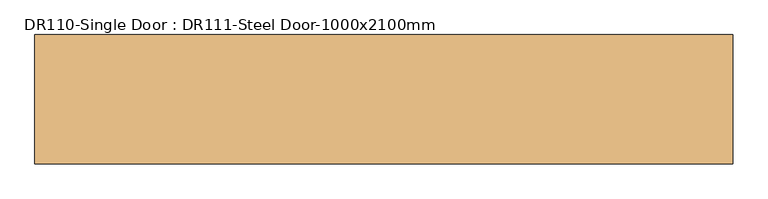
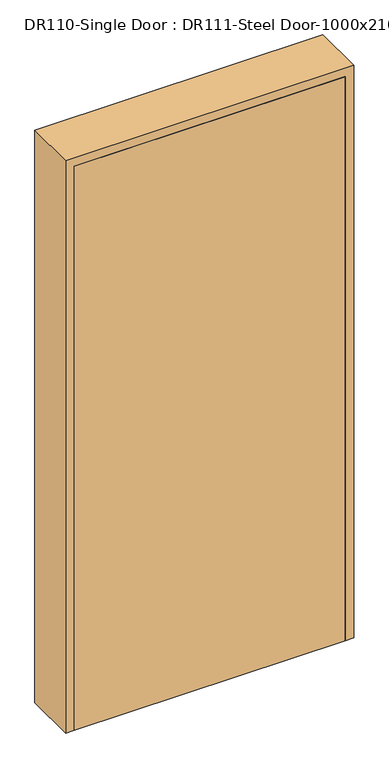
"""IFC4 building model written with IfcOpenShell, lengths in millimetres: door geometry, DR110-Single Door : DR111-Steel Door-1000x2100mm."""

from ifc_helpers import new_model, si_unit, origin, origin_with_axes, place, context, project, spatial, polyline, outline, extrude, faceted_brep, source, transform, mapped, element, save


def dr110_single_door_dr111_steel_door_1000x2100mm_67953bf6(model_context):
    return source(origin(), model_context, "Body", "SolidModel", [
        extrude(outline(polyline([(470.0, -92.5), (-470.0, -92.5), (-470.0, -57.5), (470.0, -57.5), (470.0, -92.5)])), origin_with_axes(), (0.0, 0.0, 1.0), 2070.0),
        faceted_brep([(470.0, -92.5, 0.0), (470.0, -57.5, 0.0), (450.0, -57.5, 0.0), (450.0, 57.5, 0.0), (470.0, 57.5, 0.0), (470.0, 92.5, 0.0), (500.0, 92.5, 0.0), (500.0, -92.5, 0.0), (500.0, -92.5, 2100.0), (-500.0, -92.5, 2100.0), (-500.0, -92.5, 0.0), (-470.0, -92.5, 0.0), (-470.0, -92.5, 2070.0), (470.0, -92.5, 2070.0), (500.0, 92.5, 2100.0), (470.0, 92.5, 2070.0), (-470.0, 92.5, 2070.0), (-470.0, 92.5, 0.0), (-500.0, 92.5, 0.0), (-500.0, 92.5, 2100.0), (470.0, 57.5, 2070.0), (450.0, 57.5, 2050.0), (-450.0, 57.5, 2050.0), (-450.0, 57.5, 0.0), (-470.0, 57.5, 0.0), (-470.0, 57.5, 2070.0), (450.0, -57.5, 2050.0), (470.0, -57.5, 2070.0), (-470.0, -57.5, 2070.0), (-470.0, -57.5, 0.0), (-450.0, -57.5, 0.0), (-450.0, -57.5, 2050.0)], [[[0, 1, 2, 3, 4, 5, 6, 7]], [[7, 8, 9, 10, 11, 12, 13, 0]], [[6, 14, 8, 7]], [[5, 15, 16, 17, 18, 19, 14, 6]], [[4, 20, 15, 5]], [[3, 21, 22, 23, 24, 25, 20, 4]], [[2, 26, 21, 3]], [[1, 27, 28, 29, 30, 31, 26, 2]], [[0, 13, 27, 1]], [[12, 11, 29, 28]], [[11, 10, 18, 17, 24, 23, 30, 29]], [[19, 18, 10, 9]], [[25, 24, 17, 16]], [[31, 30, 23, 22]], [[14, 19, 9, 8]], [[20, 25, 16, 15]], [[26, 31, 22, 21]], [[13, 12, 28, 27]]]),
    ])


if __name__ == "__main__":
    model = new_model("IFC4")
    model_context = context("Model", 3, world=origin())
    ifc_project = project(units=[si_unit("LENGTHUNIT", "METRE", prefix="MILLI")], contexts=[model_context])
    site = spatial("IfcSite", under=ifc_project)
    building = spatial("IfcBuilding", under=site)
    placement = place(None, origin())
    dr110_single_door_dr111_steel_door_1000x2100mm_shape = dr110_single_door_dr111_steel_door_1000x2100mm_67953bf6(model_context)
    element("IfcDoor", 1, ObjectType="DR110-Single Door : DR111-Steel Door-1000x2100mm", at=placement, inside=building, context=model_context, shape_type="MappedRepresentation", body=[
        mapped(dr110_single_door_dr111_steel_door_1000x2100mm_shape, transform((0.0, 0.0, 0.0), x_axis=(1.0, 0.0, 0.0), y_axis=(0.0, 1.0, 0.0), z_axis=(0.0, 0.0, 1.0))),
    ])
    save(model, "model.ifc")

# Revit data of these elements
# Type "DR110-Single Door : DR111-Steel Door-1000x2100mm"
#   Description = "DSDSSD"
#   Type Mark = "SD"
#   Analytic Construction = "<None>"
#   프레임 투영 외부. = 25 mm
#   프레임 투영 내부. = 25 mm
#   프레임 폭 = 75 mm
#   Height = 2100 mm
#   Width = 1000 mm
#   Define Thermal Properties by = 1
#   문 패널 = SD1 문 패널
#   문 프레임 = A04AQ098-00002_Steel Door_non FP_single
#   Function = (empty or 0)
#   Wall Closure = (empty or 0)
# Element 1 (IfcDoor, "DR110-Single Door : DR111-Steel Door-1000x2100mm")
#   Materials on its faces: "A04AQ098-00002_Steel Door_non FP_single", "SD1 문 패널"
# Materials
#   "SD1 문 패널": class "금속", colour RGB 247 247 247, transparency 0, Description = "STEEL DOOR (1000Wx2100H)"
#   "A04AQ098-00002_Steel Door_non FP_single": class "금속", colour RGB 247 247 247, transparency 0, Description = "Steel Door", W00) Work Master Code = "A04AQ098-00002", W01) Work Master_Lv1 = "Finishing Work", W02) Work Master_Lv2 = "Door & Window Work", W03) Work Master_Spec.1 = "Steel Door w/ Steel Frame", W04) Work Master_Spec.2 = "Fire Protective Rating: N/A, Single Door", W05) Work Master_Spec.3 = "w/ Hardware & Accessories", Cost = 0
